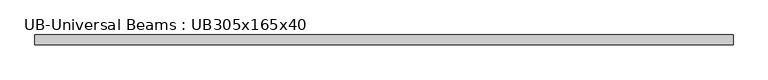
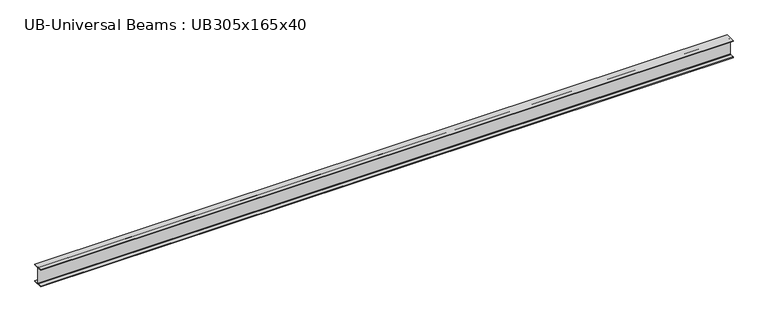
"""IFC4 building model written with IfcOpenShell, lengths in millimetres: member geometry, UB-Universal Beams : UB305x165x40."""

from ifc_helpers import new_model, si_unit, point, frame, frame_2d, origin, place, context, project, spatial, polyline, circle_curve, trimmed, segment, composite_curve, outline, extrude, source, transform, mapped, element, save


def ub_universal_beams_ub305x165x40_783ac592(model_context):
    return source(origin(), model_context, "Body", "SweptSolid", [
        extrude(outline(composite_curve([segment(polyline([(82.5, -141.5), (82.5, -151.7), (-82.5, -151.7), (-82.5, -141.5), (-11.9, -141.5)]), True, "CONTINUOUS"), segment(trimmed(circle_curve(frame_2d((-11.9, -132.6)), 8.9), [point((-11.9, -141.5))], [point((-3.0, -132.6))], True, "CARTESIAN"), True, "CONTINUOUS"), segment(polyline([(-3.0, -132.6), (-3.0, 132.6)]), True, "CONTINUOUS"), segment(trimmed(circle_curve(frame_2d((-11.9, 132.6)), 8.9), [point((-3.0, 132.6))], [point((-11.9, 141.5))], True, "CARTESIAN"), True, "CONTINUOUS"), segment(polyline([(-11.9, 141.5), (-82.5, 141.5), (-82.5, 151.7), (82.5, 151.7), (82.5, 141.5), (11.9, 141.5)]), True, "CONTINUOUS"), segment(trimmed(circle_curve(frame_2d((11.9, 132.6)), 8.9), [point((11.9, 141.5))], [point((3.0, 132.6))], True, "CARTESIAN"), True, "CONTINUOUS"), segment(polyline([(3.0, 132.6), (3.0, -132.6)]), True, "CONTINUOUS"), segment(trimmed(circle_curve(frame_2d((11.9, -132.6)), 8.9), [point((3.0, -132.6))], [point((11.9, -141.5))], True, "CARTESIAN"), True, "CONTINUOUS"), segment(polyline([(11.9, -141.5), (82.5, -141.5)]), True, "CONTINUOUS")], self_intersect=False)), frame((-5697.7, 0.0, 0.0), z_axis=(1.0, 0.0, 0.0), x_axis=(0.0, 1.0, 0.0)), (0.0, 0.0, 1.0), 11670.0),
    ])


if __name__ == "__main__":
    model = new_model("IFC4")
    model_context = context("Model", 3, world=origin())
    ifc_project = project(units=[si_unit("LENGTHUNIT", "METRE", prefix="MILLI")], contexts=[model_context])
    site = spatial("IfcSite", under=ifc_project)
    building = spatial("IfcBuilding", under=site)
    placement = place(None, origin())
    ub_universal_beams_ub305x165x40_shape = ub_universal_beams_ub305x165x40_783ac592(model_context)
    element("IfcMember", 1, ObjectType="UB-Universal Beams : UB305x165x40", at=placement, inside=building, context=model_context, shape_type="MappedRepresentation", body=[
        mapped(ub_universal_beams_ub305x165x40_shape, transform((0.0, 0.0, 0.0), x_axis=(1.0, 0.0, 0.0), y_axis=(0.0, 1.0, 0.0), z_axis=(0.0, 0.0, 1.0))),
    ])
    save(model, "model.ifc")

# Revit data of these elements
# Type "UB-Universal Beams : UB305x165x40"
#   Section Name Key = "UB305X165X40"
#   Width = 16.5 cm
#   Web Thickness = 0.6 cm
#   Web Fillet = 0.89 cm
#   Warping Constant = 164000.0 cm⁶
#   Torsional Moment of Inertia = 14.70 cm⁴
#   Section Area = 51.3 cm²
#   Plastic Modulus weak axis = 142.0 cm³
#   Plastic Modulus strong axis = 623.0 cm³
#   Nominal Weight = 40.2999 kgf/m
#   Moment of Inertia weak axis = 764.00 cm⁴
#   Moment of Inertia strong axis = 8503.00 cm⁴
#   Height = 30.34 cm
#   Flange Thickness = 1.02 cm
#   Elastic Modulus weak axis = 92.6 cm³
#   Elastic Modulus strong axis = 560.0 cm³
#   Centroid Vertical = 15.17 cm
#   Centroid Horizontal = 8.25 cm
#   Bolt Spacing = 9.0 cm
#   Length [instance default] = 1500 mm
#   Structural Material [instance default] = Metal - Steel 43-275
#   Type Comments = ""
#   Assembly Code = ""
# Element 1 (IfcMember, "UB-Universal Beams : UB305x165x40")
#   Materials on its faces: "Metal - Steel 43-275"
# Materials
#   "Metal - Steel 43-275": class "Metal", colour RGB 247 247 247, transparency 0, Cost = 0
